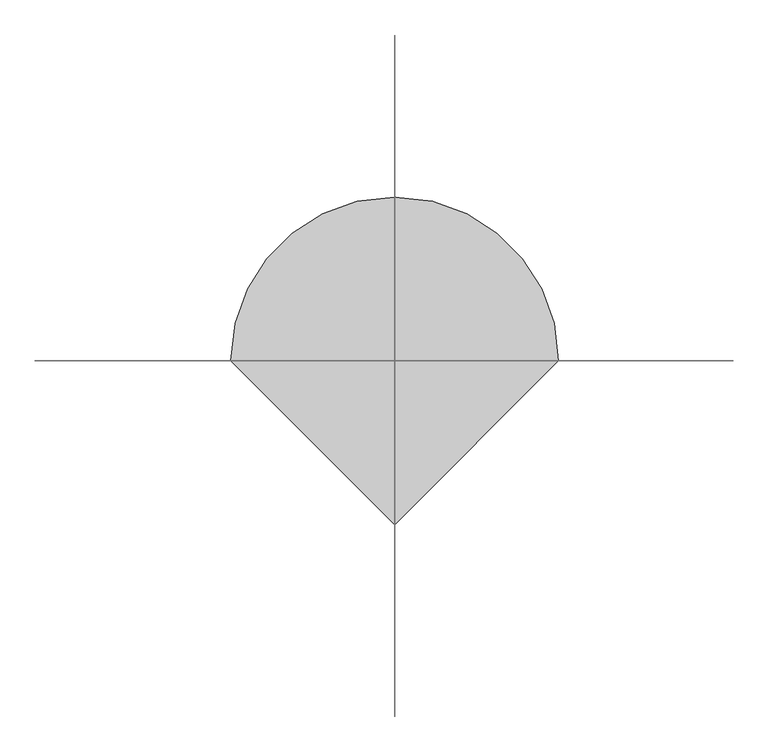
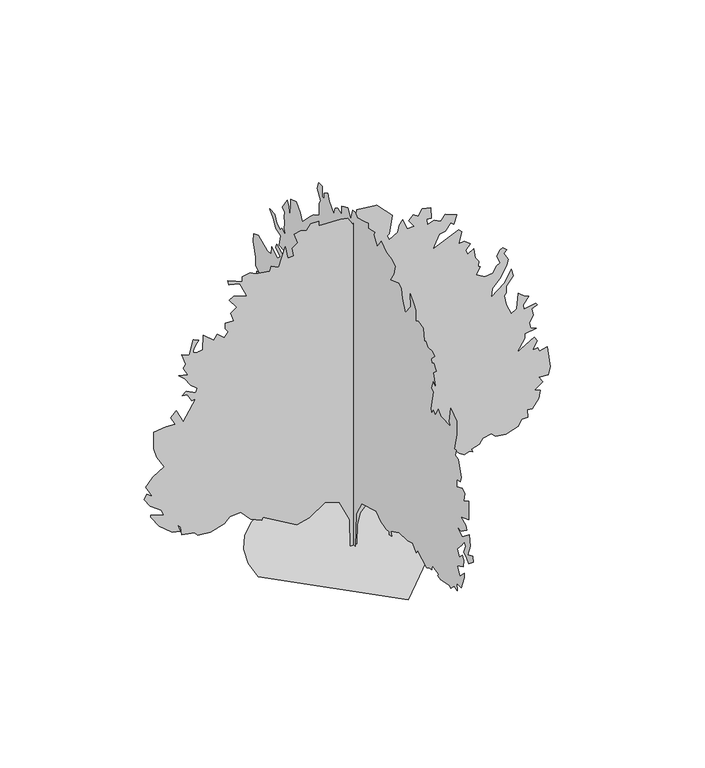
"""IFC4 building model written with IfcOpenShell, lengths in millimetres: proxy geometry, daphne 26070 : daphne 26070."""

from ifc_helpers import new_model, si_unit, origin, place, context, project, spatial, triangles, source, transform, mapped, element, save


def entourage_98a115af(model_context):
    return source(origin(), model_context, "Body", "Tessellation", [
        triangles([(-9.4573925, 3.9e-06, 72.2348623), (-36.4693492, 6.1e-06, 128.8771626), (-74.629579, 5.2e-06, 141.2324949), (-113.9485589, 1.8e-06, 114.0498972), (-145.9624841, -1e-07, 106.0463523), (-234.001251, -8e-07, 158.0691489), (-236.002001, -1.4e-06, 150.0658583), (-264.0154255, -1.9e-06, 162.0709213), (-290.0250479, -1.3e-06, 190.0833467), (-318.0387268, -2.7e-06, 188.0823242), (-332.0443036, -4.1e-06, 174.0762387), (-368.4272936, -6.4e-06, 163.6409018), (-400.0731817, -7.6e-06, 166.0726938), (-408.0767266, -7.3e-06, 176.0772612), (-442.0924192, -8.5e-06, 182.0797836), (-444.0939686, -7.2e-06, 204.089414), (-452.0975135, -7.1e-06, 212.0929589), (-446.0929381, -7.9e-06, 194.0851191), (-466.1030903, -8.6e-06, 198.0868916), (-500.1187829, -8.4e-06, 226.0990444), (-522.1279046, -7.4e-06, 258.1124609), (-522.1279046, -7.1e-06, 264.1170363), (-488.1121757, -6.3e-06, 252.1104472), (-494.1142076, -5.6e-06, 268.117537), (-522.9229142, -5.6e-06, 288.9353979), (-538.1349944, -4.9e-06, 312.1357804), (-532.1304191, -3.9e-06, 324.1423513), (-518.1248423, -3.9e-06, 314.1372934), (-534.1319321, -2.8e-06, 344.14996), (-516.6084741, -8e-07, 365.2878413), (-486.7989927, 1.6e-06, 383.4742676), (-506.1208148, 2.7e-06, 416.1818642), (-514.1243597, 3.9e-06, 442.1940482), (-514.1243597, 6.5e-06, 486.2122553), (-482.1101801, 8.1e-06, 490.2153176), (-458.099509, 9.1e-06, 488.2138046), (-470.1035728, 9.9e-06, 510.2229263), (-456.097996, 1.13e-05, 524.2284668), (-438.0893932, 1e-05, 488.2138046), (-406.0752136, 1.45e-05, 540.2355566), (-416.0802715, 1.39e-05, 538.236587), (-428.0868788, 1.46e-05, 558.2441957), (-440.0909062, 1.42e-05, 560.2457088), (-430.0883918, 1.51e-05, 568.2492537), (-406.0752136, 1.54e-05, 556.2426827), (-401.4955876, 1.62e-05, 567.0275259), (-418.0817845, 1.63e-05, 580.2533175), (-434.0888743, 1.7e-05, 604.2639522), (-450.0959641, 1.72e-05, 618.2720724), (-426.0853294, 1.79e-05, 612.2674971), (-438.0893932, 1.87e-05, 634.2791622), (-432.0873613, 1.94e-05, 642.2826708), (-442.0924192, 2.07e-05, 672.2953737), (-422.0823034, 2.11e-05, 664.2917925), (-412.0797526, 2.38e-05, 702.308004), (-398.0716687, 2.41e-05, 696.3059721), (-400.6802304, 2.38e-05, 693.2783226), (-403.212634, 2.35e-05, 690.2023476), (-405.5926123, 2.32e-05, 687.0248526), (-407.7439708, 2.29e-05, 683.6948959), (-409.5930948, 2.26e-05, 680.1642975), (-411.0637536, 2.23e-05, 676.3821882), (-412.0797526, 2.21e-05, 672.2953737), (-411.9857903, 2.19e-05, 668.7317104), (-410.3525688, 2.18e-05, 666.420369), (-407.434106, 2.18e-05, 665.1452288), (-403.4920137, 2.2e-05, 664.7033226), (-398.7777666, 2.22e-05, 664.8861603), (-393.5530128, 2.25e-05, 665.485615), (-388.0691179, 2.28e-05, 666.2907984), (-386.0676049, 2.52e-05, 706.3085592), (-360.0554572, 2.49e-05, 682.2978882), (-350.0529064, 2.62e-05, 696.3059721), (-332.0443036, 2.6e-05, 680.2988823), (-322.0392457, 2.72e-05, 692.3029461), (-330.0427906, 2.76e-05, 704.3095533), (-330.0427906, 2.84e-05, 718.3150938), (-308.0336689, 2.94e-05, 718.3150938), (-316.0372138, 3.03e-05, 740.3242155), (-301.0029389, 3.16e-05, 751.5637184), (-320.0377327, 3.24e-05, 778.340427), (-308.0336689, 3.33e-05, 784.3424589), (-274.0179581, 3.42e-05, 774.3399445), (-292.0265791, 3.57e-05, 812.356156), (-320.9191106, 3.49e-05, 820.7254852), (-324.0407587, 3.54e-05, 832.3637283), (-304.0306247, 3.58e-05, 824.3602198), (-286.0245472, 3.62e-05, 816.3566385), (-286.0245472, 3.7e-05, 830.3647951), (-265.0619096, 3.8e-05, 832.6329706), (-252.0090908, 3.82e-05, 826.3616964), (-215.9931387, 3.95e-05, 820.3596645), (-211.9913662, 4.03e-05, 832.3637283), (-191.9827583, 4.06e-05, 822.3612139), (-175.9756504, 4.43e-05, 872.3814892), (-168.7203883, 4.27e-05, 839.3385933), (-153.9660381, 4.34e-05, 840.3673096), (-157.9678106, 4.45e-05, 862.3789747), (-143.9617251, 4.57e-05, 872.3814892), (-151.9650156, 4.69e-05, 898.3936369), (-135.9581802, 4.78e-05, 902.3941195), (-119.9513447, 4.83e-05, 898.3936369), (-109.9467864, 4.96e-05, 912.3991774), (-89.9381694, 5.05e-05, 912.3991774), (-89.9381694, 4.97e-05, 900.3951862), (-32.626833, 5.21e-05, 897.7739073), (-14.3439498, 5.26e-05, 893.5625364), (-1.8993678, 5.19e-05, 872.3814892), (6.1041838, 5.31e-05, 886.3895731), (8.105045, 5.45e-05, 908.3986948), (59.627565, 5.65e-05, 903.8140182), (99.4230465, 5.58e-05, 862.5999641), (92.1418776, 5.26e-05, 814.3577053), (86.1393461, 5.21e-05, 810.3546066), (92.1418776, 5.16e-05, 798.3505428), (114.1514989, 5.33e-05, 810.3546066), (118.1578496, 5.45e-05, 827.9416145), (126.1568253, 5.56e-05, 840.3673096), (138.1621427, 5.45e-05, 812.356156), (155.7905089, 5.52e-05, 811.8684677), (142.1639151, 5.58e-05, 832.3637283), (154.1689872, 5.71e-05, 844.3703356), (166.1743046, 5.71e-05, 836.3667543), (176.1785995, 5.85e-05, 852.3739168), (198.1884842, 5.92e-05, 848.3708181), (200.188998, 5.75e-05, 818.3581879), (188.1839168, 5.71e-05, 820.3596645), (190.1846849, 5.63e-05, 804.3525747), (208.1927972, 5.74e-05, 810.3546066), (224.199887, 5.76e-05, 802.3510981), (236.20495, 5.9e-05, 816.3566385), (265.7807247, 5.96e-05, 805.7293076), (258.2140718, 5.79e-05, 782.343453), (250.2110355, 5.79e-05, 788.3454849), (236.20495, 5.62e-05, 770.3369184), (220.1978602, 5.54e-05, 768.3379126), (204.1910248, 5.26e-05, 732.3207069), (270.2206608, 5.73e-05, 762.3333372), (278.2242057, 5.71e-05, 754.3298286), (270.2206608, 5.5e-05, 724.3171257), (284.2262195, 5.57e-05, 726.318675), (300.2333274, 5.57e-05, 714.3120678), (288.2267384, 5.43e-05, 700.3065273), (294.2312955, 5.39e-05, 688.3024635), (309.737998, 5.51e-05, 697.179756), (312.8444218, 5.37e-05, 671.3504459), (322.242431, 5.33e-05, 658.2872171), (320.240918, 5.25e-05, 646.283226), (326.2454933, 5.25e-05, 642.2801273), (316.2403991, 5.1e-05, 624.2741043), (337.7847236, 5.12e-05, 610.9797123), (358.2596729, 5.23e-05, 614.2690464), (368.2621874, 5.37e-05, 630.2761362), (378.0386619, 5.44e-05, 634.7135107), (368.2621874, 5.52e-05, 656.2882839), (376.2657323, 5.64e-05, 670.2938244), (384.2692772, 5.7e-05, 674.2943069), (394.2743714, 5.68e-05, 664.2917925), (386.2708265, 5.61e-05, 658.2872171), (398.1707179, 5.54e-05, 637.1290609), (394.2743714, 5.43e-05, 622.272555), (376.2657323, 5.17e-05, 592.2598884), (356.2581599, 4.97e-05, 572.2497725), (354.2566106, 4.83e-05, 550.2406508), (388.2723395, 5.13e-05, 576.2527986), (406.2783989, 5.4e-05, 608.2669782), (410.2814612, 5.3e-05, 588.2568624), (392.2728221, 5.09e-05, 566.2477407), (392.2728221, 4.98e-05, 548.2391015), (388.2723395, 4.93e-05, 542.2371059), (392.2728221, 4.79e-05, 516.2249219), (406.2783989, 4.67e-05, 486.2122553), (419.6692966, 4.79e-05, 495.1530613), (424.2870017, 5.05e-05, 536.235074), (440.2941278, 5.04e-05, 522.2294972), (450.2991858, 5.06e-05, 518.2264712), (437.047996, 4.89e-05, 500.1924339), (438.2925785, 4.83e-05, 488.2138046), (468.3077886, 4.99e-05, 494.2158002), (472.3083075, 4.97e-05, 488.2138046), (458.3027307, 4.88e-05, 482.2117727), (462.5902596, 4.78e-05, 462.3895815), (452.3006988, 4.64e-05, 446.1945308), (456.3012177, 4.56e-05, 430.187441), (470.3067581, 4.58e-05, 424.1854091), (440.2941278, 4.43e-05, 420.1849265), (440.2941278, 4.36e-05, 408.1783193), (420.2865191, 4.08e-05, 376.1641397), (464.3047626, 4.43e-05, 402.1762874), (472.3083075, 4.39e-05, 390.1697165), (460.3017002, 4.21e-05, 368.1605947), (474.3098205, 4.28e-05, 370.1621078), (478.3103394, 4.24e-05, 360.1570498), (498.3204552, 4.35e-05, 364.1600759), (506.3240001, 4.05e-05, 308.1352615), (500.3194247, 3.9e-05, 288.1251276), (476.3113335, 3.81e-05, 290.1266587), (486.3138843, 3.76e-05, 274.1195508), (464.3047626, 3.57e-05, 258.1124609), (480.3118524, 3.6e-05, 252.1104472), (476.3113335, 3.47e-05, 232.1015668), (460.3017002, 3.26e-05, 210.0919546), (446.2961234, 3.22e-05, 212.0929589), (448.2976727, 3.09e-05, 190.0833467), (432.2905829, 3.02e-05, 190.0833467), (424.2870017, 2.89e-05, 174.0762387), (391.7419679, 2.69e-05, 164.3614974), (366.2632178, 2.6e-05, 168.0737163), (354.2566106, 2.61e-05, 178.0780111), (332.2474889, 2.49e-05, 174.0762387), (323.8020015, 2.37e-05, 160.8723026), (302.2348404, 2.24e-05, 154.0673764), (306.2353412, 2.21e-05, 146.0640859), (298.2317963, 2.2e-05, 150.0658583), (284.2262195, 2.11e-05, 146.0640859), (272.2196304, 2.11e-05, 154.0673764), (260.2155848, 2.14e-05, 168.0737163), (240.2064682, 2.03e-05, 164.0719438), (236.8051496, 1.96e-05, 155.3752181), (196.1874799, 1.67e-05, 136.0595276), (196.1874799, 1.6e-05, 124.0544646), (162.1725321, 1.36e-05, 110.0481247), (162.1725321, 1.4e-05, 116.0509106), (138.1618883, 1.27e-05, 112.0491381), (106.7192036, 1.23e-05, 127.7984221), (83.214788, 1.13e-05, 128.4156446), (38.7434109, 8e-06, 104.983363), (17.3291135, 5.6e-06, 81.0641653), (9.1189377, 3.5e-06, 51.8726831), (8.1050195, 4e-07, 0.0), (-7.9020227, -3e-07, 7e-07), (-244.9072532, 0.0, 4.54e-05), (-238.4327937, 56.1165193, 4.18e-05), (-219.9933851, 107.6506239, 3.79e-05), (-191.0655541, 153.1257915, 3.39e-05), (-153.1257915, 191.0655541, 3e-05), (-107.6506239, 219.9933851, 2.63e-05), (-56.1165193, 238.4327937, 2.29e-05), (1.14e-05, 244.9072532, 2.01e-05), (56.1165193, 238.4327937, 1.8e-05), (107.6506239, 219.9933851, 5.12e-05), (153.1257915, 191.0655541, 5.1e-05), (191.0655541, 153.1257915, 5.16e-05), (219.9933851, 107.6506239, 1.87e-05), (238.4327937, 56.1165193, 2.09e-05), (244.9072532, -2.14e-05, 2.4e-05), (-3.16e-05, -244.9072532, 4.93e-05), (-1e-06, 8.7682648, 19.1210077), (-2.7e-06, 9.3654196, 78.8180451), (-6.1e-06, 33.2534526, 124.0544646), (-5.1e-06, 45.2590243, 110.0481247), (-5.2e-06, 55.2633328, 118.0516787), (-5.8e-06, 63.2666234, 112.0491381), (-6.9e-06, 91.2787853, 114.0498972), (-9e-06, 105.285116, 130.0569961), (-9.8e-06, 121.2919515, 126.0552236), (-9.6e-06, 133.2972779, 144.0630725), (-1.09e-05, 133.2972779, 162.0709213), (-1.16e-05, 181.318293, 146.0640859), (-1.37e-05, 187.3210879, 152.0666174), (-1.51e-05, 221.3357813, 154.0676308), (-1.31e-05, 215.3334951, 146.0640859), (-1.58e-05, 241.3446436, 158.0694032), (-1.53e-05, 243.3454117, 172.0754887), (-1.59e-05, 257.3504617, 172.0754887), (-1.75e-05, 259.3519928, 188.0825785), (-1.71e-05, 267.3555377, 204.089414), (-1.9e-05, 271.3585819, 214.0939814), (-1.92e-05, 297.3682044, 236.1036118), (-2.09e-05, 291.3661725, 240.1051299), (-2.09e-05, 315.3768253, 264.1170363), (-2.19e-05, 325.3818832, 250.1096791), (-2.19e-05, 331.3839151, 256.1134914), (-2.32e-05, 351.394031, 248.1086748), (-2.37e-05, 357.3960629, 242.1061342), (-2.46e-05, 381.4066976, 244.1069023), (-2.44e-05, 385.4072165, 254.1119602), (-2.53e-05, 409.4178512, 258.1124609), (-2.69e-05, 411.4193642, 272.1180377), (-2.71e-05, 423.423428, 278.1225949), (-2.96e-05, 455.4376076, 302.1332478), (-2.88e-05, 443.4335438, 310.1367745), (-3.05e-05, 469.4457278, 346.151473), (-3.18e-05, 465.4426655, 360.1570498), (-3.14e-05, 449.4355757, 354.1550179), (-3.05e-05, 445.4350931, 370.1621078), (-3.1e-05, 459.4406336, 374.1651701), (-3.29e-05, 474.5104623, 393.7968206), (-3.38e-05, 487.4517872, 434.1905033), (-3.29e-05, 443.4335438, 460.202651), (-3.07e-05, 433.4284859, 404.1778367), (-3e-05, 421.4244221, 408.1783193), (-3.36e-05, 431.6073034, 483.065209), (-3.29e-05, 419.4229091, 486.2122553), (-3.32e-05, 435.4299989, 496.2173495), (-3.43e-05, 435.4299989, 518.2264712), (-3.54e-05, 447.4340627, 554.2436769), (-3.64e-05, 443.4335438, 578.2543116), (-3.73e-05, 423.423428, 586.2578565), (-3.43e-05, 384.7290238, 566.6439737), (-3.35e-05, 367.3985773, 568.2492537), (-3.46e-05, 365.3996078, 590.2583754), (-3.2e-05, 339.38746, 574.2512856), (-3.09e-05, 325.3818832, 586.2578565), (-3.33e-05, 345.3894919, 600.2634333), (-3.26e-05, 341.388973, 610.2684912), (-3.2e-05, 313.375276, 596.2604073), (-3.12e-05, 309.3747934, 612.2674971), (-3.2e-05, 331.3839151, 614.2690464), (-3.26e-05, 324.6503509, 643.5704556), (-3.53e-05, 345.3894919, 652.2852579), (-3.49e-05, 357.3960629, 672.2953737), (-3.71e-05, 373.4031527, 688.3024635), (-3.62e-05, 351.394031, 686.3009142), (-3.44e-05, 341.388973, 668.2923477), (-3.42e-05, 327.3833962, 658.2897606), (-3.34e-05, 319.3798513, 668.2923477), (-3.31e-05, 301.3712485, 658.2897606), (-3.49e-05, 309.3747934, 674.2943069), (-3.4e-05, 305.3717311, 690.3013968), (-3.56e-05, 309.3747934, 706.3085592), (-3.5e-05, 307.3732804, 718.3150938), (-3.51e-05, 317.3783383, 726.318675), (-3.49e-05, 295.3692166, 758.3328547), (-3.52e-05, 289.3646595, 744.3272415), (-3.4e-05, 281.3610964, 716.3136171), (-3.58e-05, 279.3621268, 770.3369184), (-3.44e-05, 255.3514921, 778.340427), (-3.23e-05, 237.3428711, 760.334404), (-3.28e-05, 229.3393262, 740.3242155), (-3.11e-05, 209.330464, 760.334404), (-3.16e-05, 191.322606, 778.340427), (-3.05e-05, 177.3165205, 790.3470343), (-3.1e-05, 153.3061402, 804.3525747), (-3.17e-05, 153.3061402, 836.3667543), (-3.08e-05, 145.3025953, 848.3708181), (-3.26e-05, 161.3094307, 872.3814892), (-3.37e-05, 155.087445, 890.4942644), (-3.3e-05, 138.6373771, 891.588965), (-3.2e-05, 138.6373771, 863.4050749), (-3.17e-05, 129.7796238, 863.4050749), (-3.12e-05, 131.2962645, 876.3845152), (-3.22e-05, 115.28942, 886.3895731), (-3.04e-05, 107.2858751, 870.3824833), (-2.83e-05, 87.2770128, 848.3708181), (-2.94e-05, 81.2744813, 866.3794573), (-2.85e-05, 69.2691594, 874.3829659), (-2.82e-05, 53.2620651, 866.3794573), (-2.94e-05, 53.2620651, 888.388579), (-2.86e-05, 42.0070608, 894.8096987), (-2.75e-05, 25.2500576, 902.3966629), (-2.59e-05, 13.2446369, 878.3860645), (-2.63e-05, 3.2402807, 908.3986948), (-2.57e-05, -8.7649884, 910.4002441), (-2.58e-05, -16.768535, 900.3951862), (-2.39e-05, -50.7832783, 910.4002441), (-2.52e-05, -64.7893547, 914.4007267), (-2.37e-05, -64.7893547, 900.3951862), (-2.2e-05, -94.8025255, 908.3986948), (-2.26e-05, -90.8010074, 898.3936369), (-2.09e-05, -104.8068295, 874.3829659), (-2.11e-05, -122.8149417, 900.3951862), (-1.88e-05, -144.7590329, 883.3085838), (-1.79e-05, -169.2642141, 879.2750364), (-1.76e-05, -184.8420423, 870.3824833), (-1.68e-05, -179.1326343, 845.1882362), (-1.65e-05, -162.8324119, 820.3596645), (-1.63e-05, -200.8491321, 834.3652777), (-1.4e-05, -212.8544495, 826.3616964), (-1.49e-05, -216.8562219, 802.3510981), (-1.34e-05, -230.8623074, 772.3383951), (-1.32e-05, -254.871416, 802.3510981), (-1.4e-05, -252.8719378, 836.3667543), (-1.19e-05, -270.8810493, 816.3566385), (-1.21e-05, -276.8830812, 806.3541241), (-1.12e-05, -276.8830812, 778.340427), (-1.04e-05, -288.8871268, 784.3450024), (-9.7e-06, -310.8962485, 778.340427), (-8.7e-06, -314.8992745, 746.3262474), (-8.4e-06, -320.9013064, 748.3277967), (-6.3e-06, -330.9064007, 738.3227388), (-5.3e-06, -350.913973, 740.3242155), (-5.2e-06, -360.919031, 732.3207069), (-6.5e-06, -346.9134905, 716.3136171), (-4.7e-06, -348.9150035, 706.3085592), (-4.2e-06, -356.9185484, 710.3115852), (-4.3e-06, -368.9226122, 696.3059721), (-5.4e-06, -354.9170354, 684.2994375), (-4.1e-06, -364.9220933, 654.2867346), (-4.2e-06, -354.9170354, 662.2903158), (-3.5e-06, -346.9134905, 638.2796448), (-3.4e-06, -354.9170354, 632.2776129), (-1.8e-06, -344.9119411, 580.2533175), (-2.2e-06, -348.9150035, 568.2492537), (-1.3e-06, -354.9170354, 582.2548305), (-1.2e-06, -365.0364032, 574.0988966), (-1.8e-06, -376.9261571, 598.2619203), (4e-07, -388.932728, 586.2578565), (2.2e-06, -432.9509714, 584.2563435), (2.4e-06, -426.9489395, 594.2614014), (1e-07, -432.9509714, 634.2791622), (2.7e-06, -460.962125, 616.2705231), (3.1e-06, -458.9631191, 578.2543116), (5e-06, -448.9580612, 534.233561), (5.4e-06, -456.9616061, 534.233561), (4.5e-06, -453.2786187, 518.6607834), (5e-06, -466.966664, 516.2274653), (8e-06, -478.9707278, 474.2082278), (7.2e-06, -474.9702089, 460.202651), (6.5e-06, -460.962125, 458.201138), (7.6e-06, -458.9631191, 436.1920163), (9.3e-06, -484.9727597, 448.1960438), (9.4e-06, -495.8998544, 440.6471586), (1.04e-05, -490.9772987, 418.1833772), (9.7e-06, -512.9864204, 430.187441), (1.18e-05, -512.9864204, 380.167202), (9.6e-06, -476.9692148, 366.1616252), (1.23e-05, -498.9808436, 356.156531), (1.21e-05, -504.9828755, 346.151473), (1.23e-05, -478.9707278, 328.1428702), (1.17e-05, -462.963638, 330.1443832), (1.21e-05, -484.9727597, 316.1388064), (1.23e-05, -514.7745744, 340.233266), (1.35e-05, -520.9899653, 312.1357804), (1.38e-05, -508.9833944, 282.1231138), (1.52e-05, -530.9950596, 292.1281717), (1.67e-05, -532.7171565, 276.4538196), (1.52e-05, -513.8677983, 260.1292346), (1.52e-05, -504.9828755, 270.11905), (1.29e-05, -491.4116472, 278.5442443), (1.42e-05, -500.9798495, 300.1317166), (1.21e-05, -492.9763046, 308.1352615), (1.3e-05, -481.8053658, 291.1223283), (1.34e-05, -462.963638, 270.11905), (1.3e-05, -470.9671829, 252.1104472), (1.42e-05, -484.9727597, 266.1160058), (1.4e-05, -490.9772987, 256.1134914), (1.53e-05, -488.9757857, 238.1043617), (1.35e-05, -462.963638, 224.0982762), (1.52e-05, -472.9686959, 202.088664), (1.48e-05, -492.9763046, 222.0972719), (1.65e-05, -493.9364204, 210.9735868), (1.65e-05, -480.9722408, 176.0772612), (1.56e-05, -460.962125, 176.0772612), (1.7e-05, -462.963638, 156.0683989), (1.44e-05, -448.9580612, 160.0701714), (1.53e-05, -434.1422141, 145.3175835), (1.52e-05, -426.9489395, 150.0658583), (1.32e-05, -388.932728, 142.0623134), (1.26e-05, -374.9246078, 144.0630725), (1.31e-05, -378.9276701, 150.0658583), (1.21e-05, -350.913973, 156.0683989), (1.15e-05, -348.9150035, 144.0630725), (1.1e-05, -338.9099456, 142.0623134), (1.02e-05, -326.9033383, 136.0595276), (7.2e-06, -286.8856138, 158.0691489), (8.6e-06, -278.8845942, 148.0648449), (6.5e-06, -264.0916381, 164.6055958), (5.2e-06, -240.8666204, 158.0691489), (3.7e-06, -204.8506502, 158.0694032), (3.3e-06, -166.8341844, 138.060541), (3e-06, -170.8359568, 128.056237), (4.5e-06, -158.8306395, 124.0544646), (2.7e-06, -158.8306395, 132.0580095), (2e-06, -144.8243087, 130.0569961), (1.3e-06, -120.8141827, 138.060541), (-1e-06, -101.9528885, 154.2177488), (-2.5e-06, -36.7154756, 135.157575), (-1.1e-06, -12.638517, 93.3765678), (1.1e-06, -8.7649628, 3.52e-05), (3e-07, 9.2429405, 3.42e-05)], [[49, 48, 50], [95, 94, 96], [185, 184, 186], [213, 212, 214], [166, 165, 167], [167, 165, 168], [43, 42, 44], [53, 52, 54], [71, 70, 72], [44, 42, 45], [86, 85, 87], [85, 84, 87], [87, 84, 88], [42, 41, 45], [41, 40, 45], [174, 173, 175], [118, 117, 119], [18, 17, 19], [117, 116, 119], [145, 144, 146], [222, 221, 223], [22, 21, 23], [21, 20, 23], [133, 132, 134], [132, 131, 134], [131, 130, 134], [38, 37, 39], [37, 36, 39], [56, 55, 57], [165, 164, 168], [168, 164, 169], [169, 164, 170], [176, 175, 177], [175, 173, 177], [126, 125, 127], [180, 179, 181], [179, 178, 181], [177, 173, 178], [134, 130, 135], [135, 130, 136], [125, 124, 127], [124, 123, 127], [7, 6, 8], [27, 26, 28], [26, 25, 28], [81, 80, 82], [82, 80, 83], [158, 157, 159], [157, 156, 159], [156, 155, 159], [155, 154, 159], [159, 154, 160], [160, 154, 161], [93, 92, 94], [73, 72, 74], [204, 203, 205], [142, 141, 143], [194, 193, 195], [100, 99, 101], [57, 55, 58], [104, 103, 105], [77, 76, 78], [76, 75, 78], [110, 109, 111], [141, 140, 143], [101, 99, 102], [230, 229, 231], [231, 229, 1], [229, 228, 1], [189, 188, 190], [190, 188, 191], [198, 197, 199], [103, 102, 105], [149, 148, 150], [19, 17, 20], [20, 17, 23], [89, 88, 90], [161, 154, 162], [154, 153, 162], [153, 152, 162], [162, 152, 163], [152, 151, 163], [34, 33, 35], [1, 228, 2], [228, 227, 2], [84, 83, 88], [200, 199, 201], [48, 47, 50], [122, 121, 123], [121, 120, 123], [123, 120, 127], [127, 120, 128], [196, 195, 197], [195, 193, 197], [221, 220, 223], [192, 191, 193], [15, 14, 16], [79, 78, 80], [58, 55, 59], [55, 54, 59], [59, 54, 60], [60, 54, 61], [61, 54, 62], [62, 54, 63], [63, 54, 64], [64, 54, 65], [184, 183, 186], [130, 129, 136], [129, 128, 136], [138, 137, 139], [139, 137, 140], [88, 83, 90], [90, 83, 91], [91, 83, 92], [170, 164, 171], [29, 28, 30], [193, 191, 197], [191, 188, 197], [51, 50, 52], [25, 24, 28], [98, 97, 99], [111, 109, 112], [112, 109, 113], [113, 109, 114], [109, 108, 114], [136, 128, 137], [128, 120, 137], [202, 201, 203], [201, 199, 203], [181, 178, 182], [182, 178, 183], [35, 33, 36], [33, 32, 36], [32, 31, 36], [36, 31, 39], [120, 119, 137], [30, 28, 31], [54, 52, 65], [65, 52, 66], [52, 50, 66], [66, 50, 67], [67, 50, 68], [68, 50, 69], [119, 116, 137], [116, 115, 137], [173, 172, 178], [178, 172, 183], [183, 172, 186], [197, 188, 199], [28, 24, 31], [69, 50, 70], [215, 214, 216], [214, 212, 216], [216, 212, 217], [50, 47, 70], [47, 46, 70], [70, 46, 72], [72, 46, 74], [13, 12, 14], [206, 205, 207], [107, 106, 108], [140, 137, 143], [227, 226, 2], [147, 146, 148], [5, 4, 6], [4, 3, 6], [102, 99, 105], [99, 97, 105], [105, 97, 106], [106, 97, 108], [108, 97, 114], [114, 97, 115], [219, 218, 220], [143, 137, 144], [199, 188, 203], [203, 188, 205], [205, 188, 207], [207, 188, 208], [208, 188, 209], [209, 188, 210], [211, 210, 212], [212, 210, 217], [210, 188, 217], [217, 188, 218], [8, 6, 9], [80, 78, 83], [224, 223, 225], [223, 220, 225], [92, 83, 94], [12, 11, 14], [11, 10, 14], [14, 10, 16], [16, 10, 17], [17, 10, 23], [23, 10, 24], [24, 10, 31], [31, 10, 39], [10, 9, 39], [39, 9, 40], [9, 6, 40], [6, 3, 40], [40, 3, 45], [45, 3, 46], [46, 3, 74], [74, 3, 75], [75, 3, 78], [78, 3, 83], [83, 3, 94], [94, 3, 96], [96, 3, 97], [97, 3, 115], [115, 3, 137], [3, 2, 137], [2, 226, 137], [137, 226, 144], [144, 226, 146], [146, 226, 148], [148, 226, 150], [226, 225, 150], [225, 220, 150], [220, 218, 150], [218, 188, 150], [151, 150, 163], [163, 150, 164], [150, 188, 164], [164, 188, 171], [171, 188, 172], [172, 188, 186], [188, 187, 186], [247, 246, 232], [246, 245, 232], [232, 245, 233], [245, 244, 233], [233, 244, 234], [234, 244, 235], [244, 243, 235], [243, 242, 235], [235, 242, 236], [236, 242, 237], [237, 242, 238], [238, 242, 239], [239, 242, 240], [240, 242, 241], [262, 261, 263], [389, 388, 390], [373, 372, 374], [313, 312, 314], [441, 440, 442], [442, 440, 443], [314, 312, 315], [312, 311, 315], [359, 358, 360], [324, 323, 325], [415, 414, 416], [423, 422, 424], [302, 301, 303], [450, 449, 451], [401, 400, 402], [402, 400, 403], [400, 399, 403], [445, 444, 446], [315, 311, 316], [311, 310, 316], [290, 289, 291], [289, 288, 291], [288, 287, 291], [287, 286, 291], [281, 280, 282], [397, 396, 398], [323, 322, 325], [325, 322, 326], [463, 462, 464], [462, 461, 464], [426, 425, 427], [427, 425, 428], [428, 425, 429], [443, 440, 444], [269, 268, 270], [357, 356, 358], [395, 394, 396], [436, 435, 437], [437, 435, 438], [438, 435, 439], [429, 425, 430], [430, 425, 431], [425, 424, 431], [405, 404, 406], [374, 372, 375], [375, 372, 376], [457, 456, 458], [272, 271, 273], [372, 371, 376], [416, 414, 417], [309, 308, 310], [343, 342, 344], [342, 341, 344], [306, 305, 307], [305, 304, 307], [284, 283, 285], [283, 282, 285], [339, 338, 340], [338, 337, 340], [337, 336, 340], [362, 361, 363], [383, 382, 384], [382, 381, 384], [471, 470, 248], [470, 469, 248], [248, 469, 249], [249, 469, 250], [469, 468, 250], [387, 386, 388], [386, 385, 388], [403, 399, 404], [251, 250, 252], [351, 350, 352], [419, 418, 420], [418, 417, 420], [420, 417, 421], [322, 321, 326], [321, 320, 326], [293, 292, 294], [265, 264, 266], [317, 316, 318], [316, 310, 318], [310, 308, 318], [447, 446, 448], [431, 424, 432], [424, 422, 432], [432, 422, 433], [365, 364, 366], [278, 277, 279], [263, 261, 264], [256, 255, 257], [399, 398, 404], [327, 326, 328], [328, 326, 329], [329, 326, 330], [453, 452, 454], [398, 396, 404], [413, 412, 414], [412, 411, 414], [414, 411, 417], [378, 377, 379], [377, 376, 379], [340, 336, 341], [409, 408, 410], [344, 341, 345], [422, 421, 433], [433, 421, 434], [364, 363, 366], [366, 363, 367], [363, 361, 367], [408, 407, 410], [407, 406, 410], [392, 391, 393], [341, 336, 345], [257, 255, 258], [259, 258, 260], [380, 379, 381], [276, 275, 277], [275, 274, 277], [353, 352, 354], [354, 352, 355], [349, 348, 350], [350, 348, 352], [347, 346, 348], [346, 345, 348], [298, 297, 299], [299, 297, 300], [297, 296, 300], [295, 294, 296], [296, 294, 300], [300, 294, 301], [336, 335, 345], [335, 334, 345], [455, 454, 456], [454, 452, 456], [360, 358, 361], [368, 367, 369], [369, 367, 370], [291, 286, 292], [356, 355, 358], [449, 448, 451], [440, 439, 444], [404, 396, 406], [396, 394, 406], [406, 394, 410], [410, 394, 411], [376, 371, 379], [370, 367, 371], [301, 294, 303], [254, 253, 255], [253, 252, 255], [294, 292, 303], [319, 318, 320], [320, 318, 326], [326, 318, 330], [435, 434, 439], [355, 352, 358], [358, 352, 361], [361, 352, 367], [261, 260, 264], [417, 411, 421], [411, 394, 421], [255, 252, 258], [252, 250, 258], [352, 348, 367], [348, 345, 367], [345, 334, 367], [367, 334, 371], [334, 333, 371], [333, 332, 371], [332, 331, 371], [331, 330, 371], [330, 318, 371], [318, 308, 371], [308, 307, 371], [371, 307, 379], [379, 307, 381], [381, 307, 384], [384, 307, 385], [385, 307, 388], [388, 307, 390], [390, 307, 391], [391, 307, 393], [393, 307, 394], [394, 307, 421], [421, 307, 434], [434, 307, 439], [439, 307, 444], [444, 307, 446], [446, 307, 448], [448, 307, 451], [451, 307, 452], [452, 307, 456], [456, 307, 458], [458, 307, 459], [459, 307, 460], [460, 307, 461], [461, 307, 464], [464, 307, 465], [465, 307, 466], [466, 307, 467], [467, 307, 468], [468, 307, 250], [250, 307, 258], [307, 304, 258], [304, 303, 258], [303, 292, 258], [258, 292, 260], [274, 273, 277], [277, 273, 279], [273, 271, 279], [280, 279, 282], [279, 271, 282], [282, 271, 285], [285, 271, 286], [286, 271, 292], [292, 271, 260], [271, 270, 260], [270, 268, 260], [260, 268, 264], [264, 268, 266], [266, 268, 267]], closed=False),
    ])


if __name__ == "__main__":
    model = new_model("IFC4")
    model_context = context("Model", 3, world=origin())
    ifc_project = project(units=[si_unit("LENGTHUNIT", "METRE", prefix="MILLI")], contexts=[model_context])
    site = spatial("IfcSite", under=ifc_project)
    building = spatial("IfcBuilding", under=site)
    placement = place(None, origin())
    entourage_shape = entourage_98a115af(model_context)
    element("IfcBuildingElementProxy", 1, Name="daphne 26070 : daphne 26070", ObjectType="daphne 26070 : daphne 26070", at=placement, inside=building, context=model_context, shape_type="MappedRepresentation", body=[
        mapped(entourage_shape, transform((0.0, 0.0, 0.0), x_axis=(1.0, 0.0, 0.0), y_axis=(0.0, 1.0, 0.0), z_axis=(0.0, 0.0, 1.0))),
    ])
    save(model, "model.ifc")

# Revit data of these elements
# Type "daphne 26070 : daphne 26070"
#   built-in parameter 1005195 = "RPC-16-FUMB-EMQ0-U9RG-4000-ST1L-LVER-AU"
#   Height = 0
